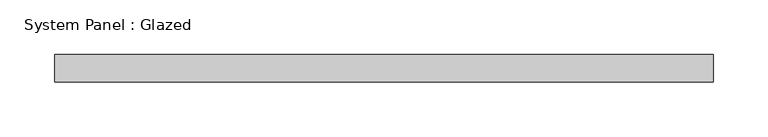
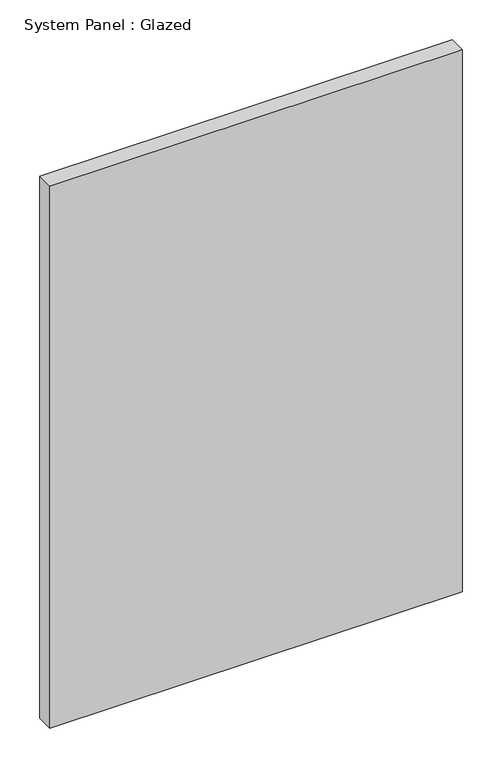
"""IFC4 building model written with IfcOpenShell, lengths in millimetres: plate geometry, System Panel : Glazed."""

from ifc_helpers import new_model, si_unit, origin, origin_with_axes, place, context, project, spatial, polyline, outline, extrude, source, transform, mapped, element, save


def system_panel_glazed_bef797c5(model_context):
    return source(origin(), model_context, "Body", "SweptSolid", [
        extrude(outline(polyline([(300.0, 24.5), (-300.0, 24.5), (-300.0, 49.5), (300.0, 49.5), (300.0, 24.5)])), origin_with_axes(), (0.0, 0.0, 1.0), 833.3333333),
    ])


if __name__ == "__main__":
    model = new_model("IFC4")
    model_context = context("Model", 3, world=origin())
    ifc_project = project(units=[si_unit("LENGTHUNIT", "METRE", prefix="MILLI")], contexts=[model_context])
    site = spatial("IfcSite", under=ifc_project)
    building = spatial("IfcBuilding", under=site)
    placement = place(None, origin())
    system_panel_glazed_shape = system_panel_glazed_bef797c5(model_context)
    element("IfcPlate", 1, ObjectType="System Panel : Glazed", at=placement, inside=building, context=model_context, shape_type="MappedRepresentation", body=[
        mapped(system_panel_glazed_shape, transform((0.0, 0.0, 0.0), x_axis=(1.0, 0.0, 0.0), y_axis=(0.0, 1.0, 0.0), z_axis=(0.0, 0.0, 1.0))),
    ])
    save(model, "model.ifc")

# Revit data of these elements
# Element 1 (IfcPlate, "System Panel : Glazed")
#   Materials on its faces: "Glass"
# Materials
#   "Glass": class "Glass", colour RGB 218 227 224, transparency 0.85, Description = "Soda Lime Glass", Cost = 0
